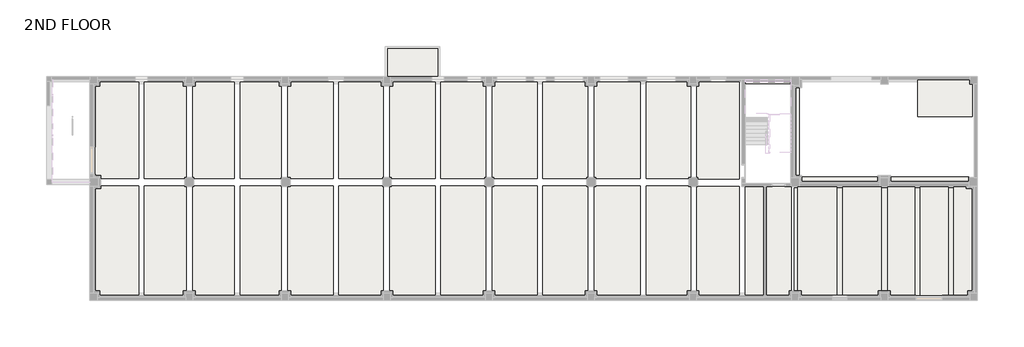
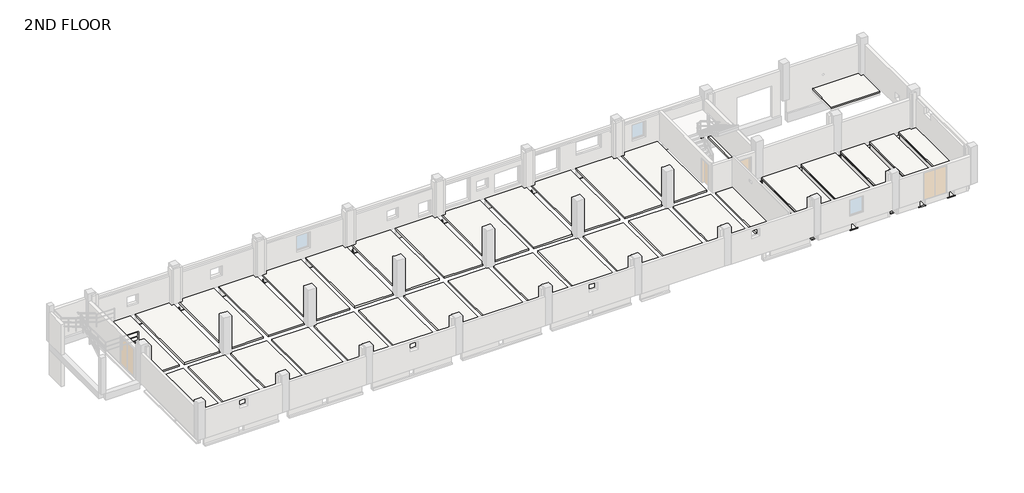
# One storey, part 4 of 7: 8 slabs, 2 coverings, 1 roof.
"""IFC4 building model written with IfcOpenShell, lengths in millimetres."""

from ifc_helpers import new_model, si_unit, frame, origin, place, context, project, spatial, polyline, outline, extrude, faceted_brep, element, save

model = new_model("IFC4")

# Units and contexts
model_context = context("Model", 3, world=origin())
ifc_project = project(units=[si_unit("LENGTHUNIT", "METRE", prefix="MILLI")], contexts=[model_context])

# Site, building, storey
site = spatial("IfcSite", under=ifc_project)
building = spatial("IfcBuilding", under=site)
storey = spatial("IfcBuildingStorey", under=building, Name="2ND FLOOR", Elevation=10600.0)

# Coverings
placement = place(None, origin())
element("IfcCovering", 1, ObjectType="H_CE_AR_B09_Souns Absorbing_100T_C7", at=placement, inside=storey, context=model_context, shape_type="SweptSolid", body=[
    extrude(outline(polyline([(58275.0, -8350.0), (58275.0, -16900.0), (55300.0, -16900.0), (55300.0, -16700.0), (55200.0, -16700.0), (55200.0, -8350.0), (58275.0, -8350.0)])), frame((0.0, 0.0, 10350.0), z_axis=(0.0, 0.0, 1.0), x_axis=(1.0, 0.0, 0.0)), (0.0, 0.0, 1.0), 100.0),
    extrude(outline(polyline([(58725.0, -8350.0), (61750.0, -8350.0), (61750.0, -16700.0), (61700.0, -16700.0), (61700.0, -16900.0), (58725.0, -16900.0), (58725.0, -8350.0)])), frame((0.0, 0.0, 10350.0), z_axis=(0.0, 0.0, 1.0), x_axis=(1.0, 0.0, 0.0)), (0.0, 0.0, 1.0), 100.0),
    extrude(outline(polyline([(64375.0, -8350.0), (64375.0, -16900.0), (62300.0, -16900.0), (62300.0, -16700.0), (62250.0, -16700.0), (62250.0, -8350.0), (64375.0, -8350.0)])), frame((0.0, 0.0, 10350.0), z_axis=(0.0, 0.0, 1.0), x_axis=(1.0, 0.0, 0.0)), (0.0, 0.0, 1.0), 100.0),
    extrude(outline(polyline([(67000.0, -8350.0), (67000.0, -16900.0), (64825.0, -16900.0), (64825.0, -8350.0), (67000.0, -8350.0)])), frame((0.0, 0.0, 10350.0), z_axis=(0.0, 0.0, 1.0), x_axis=(1.0, 0.0, 0.0)), (0.0, 0.0, 1.0), 100.0),
    extrude(outline(polyline([(68700.0, -16900.0), (67450.0, -16900.0), (67450.0, -8350.0), (68900.0, -8350.0), (68900.0, -16700.0), (68700.0, -16700.0), (68700.0, -16900.0)])), frame((0.0, 0.0, 10350.0), z_axis=(0.0, 0.0, 1.0), x_axis=(1.0, 0.0, 0.0)), (0.0, 0.0, 1.0), 100.0),
])
element("IfcCovering", 2, ObjectType="H_CE_AR_B09_Souns Absorbing_100T_C7", at=placement, inside=storey, context=model_context, shape_type="SweptSolid", body=[
    extrude(outline(polyline([(58175.0, -16886.0), (58175.0, -8469.0), (58825.0, -8469.0), (58825.0, -16886.0), (58175.0, -16886.0)])), frame((0.0, 0.0, 9700.0), z_axis=(0.0, 0.0, 1.0), x_axis=(1.0, 0.0, 0.0)), (0.0, 0.0, 1.0), 100.0),
    extrude(outline(polyline([(61650.0, -16536.0), (61650.0, -8469.0), (62350.0, -8469.0), (62350.0, -16536.0), (61650.0, -16536.0)])), frame((0.0, 0.0, 9700.0), z_axis=(0.0, 0.0, 1.0), x_axis=(1.0, 0.0, 0.0)), (0.0, 0.0, 1.0), 100.0),
    extrude(outline(polyline([(64275.0, -16886.0), (64275.0, -8469.0), (64925.0, -8469.0), (64925.0, -16886.0), (64275.0, -16886.0)])), frame((0.0, 0.0, 9700.0), z_axis=(0.0, 0.0, 1.0), x_axis=(1.0, 0.0, 0.0)), (0.0, 0.0, 1.0), 100.0),
    extrude(outline(polyline([(66900.0, -16886.0), (66900.0, -8469.0), (67550.0, -8469.0), (67550.0, -16886.0), (66900.0, -16886.0)])), frame((0.0, 0.0, 9700.0), z_axis=(0.0, 0.0, 1.0), x_axis=(1.0, 0.0, 0.0)), (0.0, 0.0, 1.0), 100.0),
    extrude(outline(polyline([(54937.0, -8469.0), (55300.0, -8469.0), (55300.0, -16536.0), (54937.0, -16536.0), (54937.0, -8469.0)])), frame((0.0, 0.0, 9700.0), z_axis=(0.0, 0.0, 1.0), x_axis=(1.0, 0.0, 0.0)), (0.0, 0.0, 1.0), 100.0),
])

# Roof
element("IfcRoof", 3, ObjectType="H_RF_AR_B06_RC Roof Finish_SkyPanel Roof_T160", at=placement, inside=storey, context=model_context, shape_type="SweptSolid", body=[
    extrude(outline(polyline([(23000.0, 2500.0), (27000.0, 2500.0), (27000.0, 300.0), (23000.0, 300.0), (23000.0, 2500.0)])), frame((0.0, 0.0, 9300.0), z_axis=(0.0, 0.0, 1.0), x_axis=(1.0, 0.0, 0.0)), (0.0, 0.0, 1.0), 170.0),
])

# Slabs
element("IfcSlab", 4, ObjectType="H_FL_AR_S17_RC Slab_T150_2S1", at=placement, inside=storey, context=model_context, shape_type="Brep", body=[
    faceted_brep([(3525.0, -100.0, 10450.0), (3525.0, -7700.0, 10450.0), (400.0, -7700.0, 10450.0), (399.4974747, -7700.0, 10450.0), (399.4974747, -7650.0, 10450.0), (100.0, -7650.0, 10450.0), (100.0, -300.0, 10450.0), (300.0, -300.0, 10450.0), (300.0, -100.0, 10450.0), (3525.0, -100.0, 10600.0), (300.0, -100.0, 10600.0), (300.0, -300.0, 10600.0), (100.0, -300.0, 10600.0), (100.0, -7650.0, 10600.0), (399.4974747, -7650.0, 10600.0), (399.4974747, -7700.0, 10600.0), (400.0, -7700.0, 10600.0), (3525.0, -7700.0, 10600.0)], [[[0, 1, 2, 3, 4, 5, 6, 7, 8]], [[9, 10, 11, 12, 13, 14, 15, 16, 17]], [[1, 0, 9, 17]], [[3, 2, 1, 17, 16, 15]], [[4, 3, 15, 14]], [[5, 4, 14, 13]], [[6, 5, 13, 12]], [[7, 6, 12, 11]], [[8, 7, 11, 10]], [[0, 8, 10, 9]]]),
    faceted_brep([(3975.0, -100.0, 10450.0), (7200.0, -100.0, 10450.0), (7200.0, -300.0, 10450.0), (7250.0, -300.0, 10450.0), (7250.0, -7650.0, 10450.0), (7150.0, -7650.0, 10450.0), (7150.0, -7700.0, 10450.0), (3975.0, -7700.0, 10450.0), (3975.0, -100.0, 10600.0), (3975.0, -7700.0, 10600.0), (7150.0, -7700.0, 10600.0), (7150.0, -7650.0, 10600.0), (7250.0, -7650.0, 10600.0), (7250.0, -300.0, 10600.0), (7200.0, -300.0, 10600.0), (7200.0, -100.0, 10600.0)], [[[0, 1, 2, 3, 4, 5, 6, 7]], [[8, 9, 10, 11, 12, 13, 14, 15]], [[1, 0, 8, 15]], [[2, 1, 15, 14]], [[3, 2, 14, 13]], [[4, 3, 13, 12]], [[5, 4, 12, 11]], [[6, 5, 11, 10]], [[7, 6, 10, 9]], [[0, 7, 9, 8]]]),
    faceted_brep([(3525.0, -16900.0, 10450.0), (300.0, -16900.0, 10450.0), (300.0, -16700.0, 10450.0), (100.0, -16700.0, 10450.0), (100.0, -8350.0, 10450.0), (399.4974747, -8350.0, 10450.0), (399.4974747, -8300.0, 10450.0), (400.0, -8300.0, 10450.0), (3525.0, -8300.0, 10450.0), (3525.0, -16900.0, 10600.0), (3525.0, -8300.0, 10600.0), (400.0, -8300.0, 10600.0), (399.4974747, -8300.0, 10600.0), (399.4974747, -8350.0, 10600.0), (100.0, -8350.0, 10600.0), (100.0, -16700.0, 10600.0), (300.0, -16700.0, 10600.0), (300.0, -16900.0, 10600.0)], [[[0, 1, 2, 3, 4, 5, 6, 7, 8]], [[9, 10, 11, 12, 13, 14, 15, 16, 17]], [[1, 0, 9, 17]], [[2, 1, 17, 16]], [[3, 2, 16, 15]], [[4, 3, 15, 14]], [[5, 4, 14, 13]], [[6, 5, 13, 12]], [[8, 7, 6, 12, 11, 10]], [[0, 8, 10, 9]]]),
    faceted_brep([(3975.0, -16900.0, 10450.0), (3975.0, -8300.0, 10450.0), (7150.0, -8300.0, 10450.0), (7150.0, -8350.0, 10450.0), (7250.0, -8350.0, 10450.0), (7250.0, -16700.0, 10450.0), (7200.0, -16700.0, 10450.0), (7200.0, -16900.0, 10450.0), (3975.0, -16900.0, 10600.0), (7200.0, -16900.0, 10600.0), (7200.0, -16700.0, 10600.0), (7250.0, -16700.0, 10600.0), (7250.0, -8350.0, 10600.0), (7150.0, -8350.0, 10600.0), (7150.0, -8300.0, 10600.0), (3975.0, -8300.0, 10600.0)], [[[0, 1, 2, 3, 4, 5, 6, 7]], [[8, 9, 10, 11, 12, 13, 14, 15]], [[1, 0, 8, 15]], [[2, 1, 15, 14]], [[3, 2, 14, 13]], [[4, 3, 13, 12]], [[5, 4, 12, 11]], [[6, 5, 11, 10]], [[7, 6, 10, 9]], [[0, 7, 9, 8]]]),
    faceted_brep([(11025.0, -100.0, 10450.0), (11025.0, -7700.0, 10450.0), (7850.0, -7700.0, 10450.0), (7850.0, -7650.0, 10450.0), (7750.0, -7650.0, 10450.0), (7750.0, -300.0, 10450.0), (7800.0, -300.0, 10450.0), (7800.0, -100.0, 10450.0), (11025.0, -100.0, 10600.0), (7800.0, -100.0, 10600.0), (7800.0, -300.0, 10600.0), (7750.0, -300.0, 10600.0), (7750.0, -7650.0, 10600.0), (7850.0, -7650.0, 10600.0), (7850.0, -7700.0, 10600.0), (11025.0, -7700.0, 10600.0)], [[[0, 1, 2, 3, 4, 5, 6, 7]], [[8, 9, 10, 11, 12, 13, 14, 15]], [[1, 0, 8, 15]], [[2, 1, 15, 14]], [[3, 2, 14, 13]], [[4, 3, 13, 12]], [[5, 4, 12, 11]], [[6, 5, 11, 10]], [[7, 6, 10, 9]], [[0, 7, 9, 8]]]),
    faceted_brep([(11025.0, -16900.0, 10450.0), (7800.0, -16900.0, 10450.0), (7800.0, -16700.0, 10450.0), (7750.0, -16700.0, 10450.0), (7750.0, -8350.0, 10450.0), (7850.0, -8350.0, 10450.0), (7850.0, -8300.0, 10450.0), (11025.0, -8300.0, 10450.0), (11025.0, -16900.0, 10600.0), (11025.0, -8300.0, 10600.0), (7850.0, -8300.0, 10600.0), (7850.0, -8350.0, 10600.0), (7750.0, -8350.0, 10600.0), (7750.0, -16700.0, 10600.0), (7800.0, -16700.0, 10600.0), (7800.0, -16900.0, 10600.0)], [[[0, 1, 2, 3, 4, 5, 6, 7]], [[8, 9, 10, 11, 12, 13, 14, 15]], [[1, 0, 8, 15]], [[2, 1, 15, 14]], [[3, 2, 14, 13]], [[4, 3, 13, 12]], [[5, 4, 12, 11]], [[6, 5, 11, 10]], [[7, 6, 10, 9]], [[0, 7, 9, 8]]]),
    faceted_brep([(14700.0, -100.0, 10450.0), (14700.0, -7700.0, 10450.0), (11475.0, -7700.0, 10450.0), (11475.0, -100.0, 10450.0), (14700.0, -100.0, 10600.0), (11475.0, -100.0, 10600.0), (11475.0, -7700.0, 10600.0), (14700.0, -7700.0, 10600.0), (14700.0, -7650.0, 10600.0), (14700.0, -300.0, 10600.0)], [[[0, 1, 2, 3]], [[4, 5, 6, 7, 8, 9]], [[1, 0, 4, 9, 8, 7]], [[2, 1, 7, 6]], [[3, 2, 6, 5]], [[0, 3, 5, 4]]]),
    faceted_brep([(11475.0, -8300.0, 10450.0), (14700.0, -8300.0, 10450.0), (14700.0, -16900.0, 10450.0), (11475.0, -16900.0, 10450.0), (11475.0, -8300.0, 10600.0), (11475.0, -16900.0, 10600.0), (14700.0, -16900.0, 10600.0), (14700.0, -16700.0, 10600.0), (14700.0, -8350.0, 10600.0), (14700.0, -8300.0, 10600.0)], [[[0, 1, 2, 3]], [[4, 5, 6, 7, 8, 9]], [[1, 0, 4, 9]], [[2, 1, 9, 8, 7, 6]], [[3, 2, 6, 5]], [[0, 3, 5, 4]]]),
    faceted_brep([(15300.0, -300.0, 10450.0), (15300.0, -100.0, 10450.0), (18775.0, -100.0, 10450.0), (18775.0, -7700.0, 10450.0), (15400.0000001, -7700.0, 10450.0), (15400.0000001, -7650.0, 10450.0), (15200.0, -7650.0, 10450.0), (15200.0, -300.0, 10450.0), (15300.0, -300.0, 10600.0), (15200.0, -300.0, 10600.0), (15200.0, -7650.0, 10600.0), (15400.0000001, -7650.0, 10600.0), (15400.0000001, -7700.0, 10600.0), (18775.0, -7700.0, 10600.0), (18775.0, -100.0, 10600.0), (15300.0, -100.0, 10600.0)], [[[0, 1, 2, 3, 4, 5, 6, 7]], [[8, 9, 10, 11, 12, 13, 14, 15]], [[1, 0, 8, 15]], [[2, 1, 15, 14]], [[3, 2, 14, 13]], [[4, 3, 13, 12]], [[5, 4, 12, 11]], [[6, 5, 11, 10]], [[7, 6, 10, 9]], [[0, 7, 9, 8]]]),
    faceted_brep([(15300.0, -16700.0, 10450.0), (15200.0, -16700.0, 10450.0), (15200.0, -8350.0, 10450.0), (15400.0000001, -8350.0, 10450.0), (15400.0000001, -8300.0, 10450.0), (18775.0, -8300.0, 10450.0), (18775.0, -16900.0, 10450.0), (15300.0, -16900.0, 10450.0), (15300.0, -16700.0, 10600.0), (15300.0, -16900.0, 10600.0), (18775.0, -16900.0, 10600.0), (18775.0, -8300.0, 10600.0), (15400.0000001, -8300.0, 10600.0), (15400.0000001, -8350.0, 10600.0), (15200.0, -8350.0, 10600.0), (15200.0, -16700.0, 10600.0)], [[[0, 1, 2, 3, 4, 5, 6, 7]], [[8, 9, 10, 11, 12, 13, 14, 15]], [[1, 0, 8, 15]], [[2, 1, 15, 14]], [[3, 2, 14, 13]], [[4, 3, 13, 12]], [[5, 4, 12, 11]], [[6, 5, 11, 10]], [[7, 6, 10, 9]], [[0, 7, 9, 8]]]),
    faceted_brep([(19225.0, -100.0, 10450.0), (22700.0, -100.0, 10450.0), (22700.0, -7650.0, 10450.0), (22650.0000003, -7650.0, 10450.0), (22650.0000003, -7700.0, 10450.0), (19225.0, -7700.0, 10450.0), (19225.0, -100.0, 10600.0), (19225.0, -7700.0, 10600.0), (22650.0000003, -7700.0, 10600.0), (22650.0000003, -7650.0, 10600.0), (22700.0, -7650.0, 10600.0), (22700.0, -300.0, 10600.0), (22700.0, -100.0, 10600.0)], [[[0, 1, 2, 3, 4, 5]], [[6, 7, 8, 9, 10, 11, 12]], [[1, 0, 6, 12]], [[2, 1, 12, 11, 10]], [[3, 2, 10, 9]], [[4, 3, 9, 8]], [[5, 4, 8, 7]], [[0, 5, 7, 6]]]),
    faceted_brep([(19225.0, -16900.0, 10450.0), (19225.0, -8300.0, 10450.0), (22650.0000003, -8300.0, 10450.0), (22650.0000003, -8350.0, 10450.0), (22700.0, -8350.0, 10450.0), (22700.0, -16900.0, 10450.0), (19225.0, -16900.0, 10600.0), (22700.0, -16900.0, 10600.0), (22700.0, -16700.0, 10600.0), (22700.0, -8350.0, 10600.0), (22650.0000003, -8350.0, 10600.0), (22650.0000003, -8300.0, 10600.0), (19225.0, -8300.0, 10600.0)], [[[0, 1, 2, 3, 4, 5]], [[6, 7, 8, 9, 10, 11, 12]], [[1, 0, 6, 12]], [[2, 1, 12, 11]], [[3, 2, 11, 10]], [[4, 3, 10, 9]], [[5, 4, 9, 8, 7]], [[0, 5, 7, 6]]]),
    faceted_brep([(23300.0, -100.0, 10450.0), (26775.0, -100.0, 10450.0), (26775.0, -7700.0, 10450.0), (23350.0000003, -7700.0, 10450.0), (23350.0000003, -7650.0, 10450.0), (23200.0, -7650.0, 10450.0), (23200.0, -300.0, 10450.0), (23300.0, -300.0, 10450.0), (23300.0, -100.0, 10600.0), (23300.0, -300.0, 10600.0), (23200.0, -300.0, 10600.0), (23200.0, -7650.0, 10600.0), (23350.0000003, -7650.0, 10600.0), (23350.0000003, -7700.0, 10600.0), (26775.0, -7700.0, 10600.0), (26775.0, -100.0, 10600.0)], [[[0, 1, 2, 3, 4, 5, 6, 7]], [[8, 9, 10, 11, 12, 13, 14, 15]], [[1, 0, 8, 15]], [[2, 1, 15, 14]], [[3, 2, 14, 13]], [[4, 3, 13, 12]], [[5, 4, 12, 11]], [[6, 5, 11, 10]], [[7, 6, 10, 9]], [[0, 7, 9, 8]]]),
    faceted_brep([(23300.0, -16900.0, 10450.0), (23300.0, -16700.0, 10450.0), (23200.0, -16700.0, 10450.0), (23200.0, -8350.0, 10450.0), (23350.0000003, -8350.0, 10450.0), (23350.0000003, -8300.0, 10450.0), (26775.0, -8300.0, 10450.0), (26775.0, -16900.0, 10450.0), (23300.0, -16900.0, 10600.0), (26775.0, -16900.0, 10600.0), (26775.0, -8300.0, 10600.0), (23350.0000003, -8300.0, 10600.0), (23350.0000003, -8350.0, 10600.0), (23200.0, -8350.0, 10600.0), (23200.0, -16700.0, 10600.0), (23300.0, -16700.0, 10600.0)], [[[0, 1, 2, 3, 4, 5, 6, 7]], [[8, 9, 10, 11, 12, 13, 14, 15]], [[1, 0, 8, 15]], [[2, 1, 15, 14]], [[3, 2, 14, 13]], [[4, 3, 13, 12]], [[5, 4, 12, 11]], [[6, 5, 11, 10]], [[7, 6, 10, 9]], [[0, 7, 9, 8]]]),
    faceted_brep([(30700.0, -100.0, 10450.0), (30700.0, -300.0, 10450.0), (30750.0000002, -300.0, 10450.0), (30750.0000002, -7650.0, 10450.0), (30649.9999997, -7650.0, 10450.0), (30649.9999997, -7700.0, 10450.0), (27225.0, -7700.0, 10450.0), (27225.0, -100.0, 10450.0), (30700.0, -100.0, 10600.0), (27225.0, -100.0, 10600.0), (27225.0, -7700.0, 10600.0), (30649.9999997, -7700.0, 10600.0), (30649.9999997, -7650.0, 10600.0), (30750.0000002, -7650.0, 10600.0), (30750.0000002, -300.0, 10600.0), (30700.0, -300.0, 10600.0)], [[[0, 1, 2, 3, 4, 5, 6, 7]], [[8, 9, 10, 11, 12, 13, 14, 15]], [[1, 0, 8, 15]], [[2, 1, 15, 14]], [[3, 2, 14, 13]], [[4, 3, 13, 12]], [[5, 4, 12, 11]], [[6, 5, 11, 10]], [[7, 6, 10, 9]], [[0, 7, 9, 8]]]),
    faceted_brep([(30700.0, -16900.0, 10450.0), (27225.0, -16900.0, 10450.0), (27225.0, -8300.0, 10450.0), (30649.9999997, -8300.0, 10450.0), (30649.9999997, -8350.0, 10450.0), (30750.0000002, -8350.0, 10450.0), (30750.0000002, -16700.0, 10450.0), (30700.0, -16700.0, 10450.0), (30700.0, -16900.0, 10600.0), (30700.0, -16700.0, 10600.0), (30750.0000002, -16700.0, 10600.0), (30750.0000002, -8350.0, 10600.0), (30649.9999997, -8350.0, 10600.0), (30649.9999997, -8300.0, 10600.0), (27225.0, -8300.0, 10600.0), (27225.0, -16900.0, 10600.0)], [[[0, 1, 2, 3, 4, 5, 6, 7]], [[8, 9, 10, 11, 12, 13, 14, 15]], [[1, 0, 8, 15]], [[2, 1, 15, 14]], [[3, 2, 14, 13]], [[4, 3, 13, 12]], [[5, 4, 12, 11]], [[6, 5, 11, 10]], [[7, 6, 10, 9]], [[0, 7, 9, 8]]]),
    faceted_brep([(31300.0, -100.0, 10450.0), (34775.0, -100.0, 10450.0), (34775.0, -7700.0, 10450.0), (31350.0000003, -7700.0, 10450.0), (31350.0000003, -7650.0, 10450.0), (31249.9999998, -7650.0, 10450.0), (31249.9999998, -300.0, 10450.0), (31300.0, -300.0, 10450.0), (31300.0, -100.0, 10600.0), (31300.0, -300.0, 10600.0), (31249.9999998, -300.0, 10600.0), (31249.9999998, -7650.0, 10600.0), (31350.0000003, -7650.0, 10600.0), (31350.0000003, -7700.0, 10600.0), (34775.0, -7700.0, 10600.0), (34775.0, -100.0, 10600.0)], [[[0, 1, 2, 3, 4, 5, 6, 7]], [[8, 9, 10, 11, 12, 13, 14, 15]], [[1, 0, 8, 15]], [[2, 1, 15, 14]], [[3, 2, 14, 13]], [[4, 3, 13, 12]], [[5, 4, 12, 11]], [[6, 5, 11, 10]], [[7, 6, 10, 9]], [[0, 7, 9, 8]]]),
    faceted_brep([(31300.0, -16900.0, 10450.0), (31300.0, -16700.0, 10450.0), (31249.9999998, -16700.0, 10450.0), (31249.9999998, -8350.0, 10450.0), (31350.0000003, -8350.0, 10450.0), (31350.0000003, -8300.0, 10450.0), (34775.0, -8300.0, 10450.0), (34775.0, -16900.0, 10450.0), (31300.0, -16900.0, 10600.0), (34775.0, -16900.0, 10600.0), (34775.0, -8300.0, 10600.0), (31350.0000003, -8300.0, 10600.0), (31350.0000003, -8350.0, 10600.0), (31249.9999998, -8350.0, 10600.0), (31249.9999998, -16700.0, 10600.0), (31300.0, -16700.0, 10600.0)], [[[0, 1, 2, 3, 4, 5, 6, 7]], [[8, 9, 10, 11, 12, 13, 14, 15]], [[1, 0, 8, 15]], [[2, 1, 15, 14]], [[3, 2, 14, 13]], [[4, 3, 13, 12]], [[5, 4, 12, 11]], [[6, 5, 11, 10]], [[7, 6, 10, 9]], [[0, 7, 9, 8]]]),
    faceted_brep([(38700.0, -100.0, 10450.0), (38700.0, -300.0, 10450.0), (38750.0000002, -300.0, 10450.0), (38750.0000002, -7650.0, 10450.0), (38649.9999997, -7650.0, 10450.0), (38649.9999997, -7700.0, 10450.0), (35225.0, -7700.0, 10450.0), (35225.0, -100.0, 10450.0), (38700.0, -100.0, 10600.0), (35225.0, -100.0, 10600.0), (35225.0, -7700.0, 10600.0), (38649.9999997, -7700.0, 10600.0), (38649.9999997, -7650.0, 10600.0), (38750.0000002, -7650.0, 10600.0), (38750.0000002, -300.0, 10600.0), (38700.0, -300.0, 10600.0)], [[[0, 1, 2, 3, 4, 5, 6, 7]], [[8, 9, 10, 11, 12, 13, 14, 15]], [[1, 0, 8, 15]], [[2, 1, 15, 14]], [[3, 2, 14, 13]], [[4, 3, 13, 12]], [[5, 4, 12, 11]], [[6, 5, 11, 10]], [[7, 6, 10, 9]], [[0, 7, 9, 8]]]),
    faceted_brep([(38700.0, -16900.0, 10450.0), (35225.0, -16900.0, 10450.0), (35225.0, -8300.0, 10450.0), (38649.9999997, -8300.0, 10450.0), (38649.9999997, -8350.0, 10450.0), (38750.0000002, -8350.0, 10450.0), (38750.0000002, -16700.0, 10450.0), (38700.0, -16700.0, 10450.0), (38700.0, -16900.0, 10600.0), (38700.0, -16700.0, 10600.0), (38750.0000002, -16700.0, 10600.0), (38750.0000002, -8350.0, 10600.0), (38649.9999997, -8350.0, 10600.0), (38649.9999997, -8300.0, 10600.0), (35225.0, -8300.0, 10600.0), (35225.0, -16900.0, 10600.0)], [[[0, 1, 2, 3, 4, 5, 6, 7]], [[8, 9, 10, 11, 12, 13, 14, 15]], [[1, 0, 8, 15]], [[2, 1, 15, 14]], [[3, 2, 14, 13]], [[4, 3, 13, 12]], [[5, 4, 12, 11]], [[6, 5, 11, 10]], [[7, 6, 10, 9]], [[0, 7, 9, 8]]]),
    faceted_brep([(39300.0, -100.0, 10450.0), (42875.0, -100.0, 10450.0), (42875.0, -7700.0, 10450.0), (39350.0000003, -7700.0, 10450.0), (39350.0000003, -7650.0, 10450.0), (39249.9999998, -7650.0, 10450.0), (39249.9999998, -300.0, 10450.0), (39300.0, -300.0, 10450.0), (39300.0, -100.0, 10600.0), (39300.0, -300.0, 10600.0), (39249.9999998, -300.0, 10600.0), (39249.9999998, -7650.0, 10600.0), (39350.0000003, -7650.0, 10600.0), (39350.0000003, -7700.0, 10600.0), (42875.0, -7700.0, 10600.0), (42875.0, -100.0, 10600.0)], [[[0, 1, 2, 3, 4, 5, 6, 7]], [[8, 9, 10, 11, 12, 13, 14, 15]], [[1, 0, 8, 15]], [[2, 1, 15, 14]], [[3, 2, 14, 13]], [[4, 3, 13, 12]], [[5, 4, 12, 11]], [[6, 5, 11, 10]], [[7, 6, 10, 9]], [[0, 7, 9, 8]]]),
    faceted_brep([(39300.0, -16900.0, 10450.0), (39300.0, -16700.0, 10450.0), (39249.9999998, -16700.0, 10450.0), (39249.9999998, -8350.0, 10450.0), (39350.0000003, -8350.0, 10450.0), (39350.0000003, -8300.0, 10450.0), (42875.0, -8300.0, 10450.0), (42875.0, -16900.0, 10450.0), (39300.0, -16900.0, 10600.0), (42875.0, -16900.0, 10600.0), (42875.0, -8300.0, 10600.0), (39350.0000003, -8300.0, 10600.0), (39350.0000003, -8350.0, 10600.0), (39249.9999998, -8350.0, 10600.0), (39249.9999998, -16700.0, 10600.0), (39300.0, -16700.0, 10600.0)], [[[0, 1, 2, 3, 4, 5, 6, 7]], [[8, 9, 10, 11, 12, 13, 14, 15]], [[1, 0, 8, 15]], [[2, 1, 15, 14]], [[3, 2, 14, 13]], [[4, 3, 13, 12]], [[5, 4, 12, 11]], [[6, 5, 11, 10]], [[7, 6, 10, 9]], [[0, 7, 9, 8]]]),
    faceted_brep([(46700.0, -100.0, 10450.0), (46700.0, -300.0, 10450.0), (46800.0, -300.0, 10450.0), (46800.0, -7650.0, 10450.0), (46649.9999999, -7650.0, 10450.0), (46649.9999999, -7700.0, 10450.0), (43325.0, -7700.0, 10450.0), (43325.0, -100.0, 10450.0), (46700.0, -100.0, 10600.0), (43325.0, -100.0, 10600.0), (43325.0, -7700.0, 10600.0), (46649.9999999, -7700.0, 10600.0), (46649.9999999, -7650.0, 10600.0), (46800.0, -7650.0, 10600.0), (46800.0, -300.0, 10600.0), (46700.0, -300.0, 10600.0)], [[[0, 1, 2, 3, 4, 5, 6, 7]], [[8, 9, 10, 11, 12, 13, 14, 15]], [[1, 0, 8, 15]], [[2, 1, 15, 14]], [[3, 2, 14, 13]], [[4, 3, 13, 12]], [[5, 4, 12, 11]], [[6, 5, 11, 10]], [[7, 6, 10, 9]], [[0, 7, 9, 8]]]),
    faceted_brep([(46700.0, -16900.0, 10450.0), (43325.0, -16900.0, 10450.0), (43325.0, -8300.0, 10450.0), (46649.9999999, -8300.0, 10450.0), (46649.9999999, -8350.0, 10450.0), (46800.0, -8350.0, 10450.0), (46800.0, -16700.0, 10450.0), (46700.0, -16700.0, 10450.0), (46700.0, -16900.0, 10600.0), (46700.0, -16700.0, 10600.0), (46800.0, -16700.0, 10600.0), (46800.0, -8350.0, 10600.0), (46649.9999999, -8350.0, 10600.0), (46649.9999999, -8300.0, 10600.0), (43325.0, -8300.0, 10600.0), (43325.0, -16900.0, 10600.0)], [[[0, 1, 2, 3, 4, 5, 6, 7]], [[8, 9, 10, 11, 12, 13, 14, 15]], [[1, 0, 8, 15]], [[2, 1, 15, 14]], [[3, 2, 14, 13]], [[4, 3, 13, 12]], [[5, 4, 12, 11]], [[6, 5, 11, 10]], [[7, 6, 10, 9]], [[0, 7, 9, 8]]]),
    faceted_brep([(50625.0, -8350.0, 10450.0), (50625.0, -16900.0, 10450.0), (47300.0, -16900.0, 10450.0), (47300.0, -8350.0, 10450.0), (50625.0, -8350.0, 10600.0), (47349.9999999, -8350.0, 10600.0), (47300.0, -8350.0, 10600.0), (47300.0, -16700.0, 10600.0), (47300.0, -16900.0, 10600.0), (50625.0, -16900.0, 10600.0)], [[[0, 1, 2, 3]], [[4, 5, 6, 7, 8, 9]], [[1, 0, 4, 9]], [[2, 1, 9, 8]], [[3, 2, 8, 7, 6]], [[0, 3, 6, 5, 4]]]),
    faceted_brep([(50625.0, -100.0, 10450.0), (50625.0, -7750.0, 10450.0), (47349.9999999, -7750.0, 10450.0), (47349.9999999, -7650.0, 10450.0), (47300.0, -7650.0, 10450.0), (47300.0, -100.0, 10450.0), (50625.0, -100.0, 10600.0), (47300.0, -100.0, 10600.0), (47300.0, -300.0, 10600.0), (47300.0, -7650.0, 10600.0), (47349.9999999, -7650.0, 10600.0), (47349.9999999, -7750.0, 10600.0), (50625.0, -7750.0, 10600.0)], [[[0, 1, 2, 3, 4, 5]], [[6, 7, 8, 9, 10, 11, 12]], [[1, 0, 6, 12]], [[2, 1, 12, 11]], [[3, 2, 11, 10]], [[4, 3, 10, 9]], [[5, 4, 9, 8, 7]], [[0, 5, 7, 6]]]),
    faceted_brep([(54700.0, -8350.0, 10450.0), (54700.0, -16900.0, 10450.0), (51075.0, -16900.0, 10450.0), (51075.0, -8350.0, 10450.0), (54700.0, -8350.0, 10600.0), (54650.0, -8350.0, 10600.0), (51075.0, -8350.0, 10600.0), (51075.0, -16900.0, 10600.0), (54700.0, -16900.0, 10600.0), (54700.0, -16700.0, 10600.0)], [[[0, 1, 2, 3]], [[4, 5, 6, 7, 8, 9]], [[1, 0, 4, 9, 8]], [[2, 1, 8, 7]], [[3, 2, 7, 6]], [[0, 3, 6, 5, 4]]]),
    faceted_brep([(58275.0, -8350.0, 10450.0), (58275.0, -16900.0, 10450.0), (55300.0, -16900.0, 10450.0), (55300.0, -16700.0, 10450.0), (55200.0, -16700.0, 10450.0), (55200.0, -8350.0, 10450.0), (58275.0, -8350.0, 10600.0), (55350.0, -8350.0, 10600.0), (55200.0, -8350.0, 10600.0), (55200.0, -16700.0, 10600.0), (55300.0, -16700.0, 10600.0), (55300.0, -16900.0, 10600.0), (58275.0, -16900.0, 10600.0)], [[[0, 1, 2, 3, 4, 5]], [[6, 7, 8, 9, 10, 11, 12]], [[1, 0, 6, 12]], [[2, 1, 12, 11]], [[3, 2, 11, 10]], [[4, 3, 10, 9]], [[5, 4, 9, 8]], [[0, 5, 8, 7, 6]]]),
    faceted_brep([(58725.0, -8350.0, 10450.0), (61750.0, -8350.0, 10450.0), (61750.0, -16700.0, 10450.0), (61700.0, -16700.0, 10450.0), (61700.0, -16900.0, 10450.0), (58725.0, -16900.0, 10450.0), (58725.0, -8350.0, 10600.0), (58725.0, -16900.0, 10600.0), (61700.0, -16900.0, 10600.0), (61700.0, -16700.0, 10600.0), (61750.0, -16700.0, 10600.0), (61750.0, -8350.0, 10600.0), (61650.0, -8350.0, 10600.0)], [[[0, 1, 2, 3, 4, 5]], [[6, 7, 8, 9, 10, 11, 12]], [[1, 0, 6, 12, 11]], [[2, 1, 11, 10]], [[3, 2, 10, 9]], [[4, 3, 9, 8]], [[5, 4, 8, 7]], [[0, 5, 7, 6]]]),
    faceted_brep([(64375.0, -8350.0, 10450.0), (64375.0, -16900.0, 10450.0), (62300.0, -16900.0, 10450.0), (62300.0, -16700.0, 10450.0), (62250.0, -16700.0, 10450.0), (62250.0, -8350.0, 10450.0), (64375.0, -8350.0, 10600.0), (62350.0, -8350.0, 10600.0), (62250.0, -8350.0, 10600.0), (62250.0, -16700.0, 10600.0), (62300.0, -16700.0, 10600.0), (62300.0, -16900.0, 10600.0), (64375.0, -16900.0, 10600.0)], [[[0, 1, 2, 3, 4, 5]], [[6, 7, 8, 9, 10, 11, 12]], [[1, 0, 6, 12]], [[2, 1, 12, 11]], [[3, 2, 11, 10]], [[4, 3, 10, 9]], [[5, 4, 9, 8]], [[0, 5, 8, 7, 6]]]),
    faceted_brep([(67000.0, -8350.0, 10450.0), (67000.0, -16900.0, 10450.0), (64825.0, -16900.0, 10450.0), (64825.0, -8350.0, 10450.0), (67000.0, -8350.0, 10600.0), (64825.0, -8350.0, 10600.0), (64825.0, -16900.0, 10600.0), (67000.0, -16900.0, 10600.0)], [[[0, 1, 2, 3]], [[4, 5, 6, 7]], [[1, 0, 4, 7]], [[2, 1, 7, 6]], [[3, 2, 6, 5]], [[0, 3, 5, 4]]]),
    faceted_brep([(68700.0, -16900.0, 10450.0), (67450.0, -16900.0, 10450.0), (67450.0, -8350.0, 10450.0), (68900.0, -8350.0, 10450.0), (68900.0, -16700.0, 10450.0), (68700.0, -16700.0, 10450.0), (68700.0, -16900.0, 10600.0), (68700.0, -16700.0, 10600.0), (68900.0, -16700.0, 10600.0), (68900.0, -8350.0, 10600.0), (68600.0, -8350.0, 10600.0), (67450.0, -8350.0, 10600.0), (67450.0, -16900.0, 10600.0)], [[[0, 1, 2, 3, 4, 5]], [[6, 7, 8, 9, 10, 11, 12]], [[1, 0, 6, 12]], [[2, 1, 12, 11]], [[3, 2, 11, 10, 9]], [[4, 3, 9, 8]], [[5, 4, 8, 7]], [[0, 5, 7, 6]]]),
])
element("IfcSlab", 5, ObjectType="H_FL_AR_S17_RC Slab_T150_2S2", at=placement, inside=storey, context=model_context, shape_type="SweptSolid", body=[
    extrude(outline(polyline([(68900.0, -2850.0), (64600.0, -2850.0), (64600.0, 50.0), (68700.0, 50.0), (68700.0, -300.0), (68900.0, -300.0), (68900.0, -2850.0)])), frame((0.0, 0.0, 10450.0), z_axis=(0.0, 0.0, 1.0), x_axis=(1.0, 0.0, 0.0)), (0.0, 0.0, 1.0), 150.0),
])
element("IfcSlab", 6, ObjectType="H_FL_AR_S17_RC Slab_T150_2CS1", at=placement, inside=storey, context=model_context, shape_type="SweptSolid", body=[
    extrude(outline(polyline([(26850.0, 2350.0), (26850.0, 300.0), (23150.0, 300.0), (23150.0, 2350.0), (26850.0, 2350.0)])), frame((0.0, 0.0, 9150.0), z_axis=(0.0, 0.0, 1.0), x_axis=(1.0, 0.0, 0.0)), (0.0, 0.0, 1.0), 150.0),
])
element("IfcSlab", 7, ObjectType="H_FL_AR_B07l_2L Gypsum_Insulationl_T154", at=placement, inside=storey, context=model_context, shape_type="Brep", body=[
    faceted_brep([(54910.0, -7486.0, 10600.0), (54910.0, -564.0, 10600.0), (55160.0, -564.0, 10600.0), (55160.0, -7486.0, 10600.0), (55314.0, -564.0, 10754.0), (55064.0, -564.0, 10754.0), (54910.0, -564.0, 10754.0), (54910.0, -7486.0, 10754.0), (55064.0, -7486.0, 10754.0), (55314.0, -7486.0, 10754.0), (55314.0, -564.0, 10735.0), (55160.0, -564.0, 10735.0), (55314.0, -7486.0, 10735.0), (54910.0, -7486.0, 10735.0), (55160.0, -7486.0, 10735.0)], [[[0, 1, 2, 3]], [[4, 5, 6, 7, 8, 9]], [[6, 5, 4, 10, 11, 2, 1]], [[4, 9, 12, 10]], [[9, 8, 7, 13, 0, 3, 14, 12]], [[1, 0, 13, 7, 6]], [[11, 14, 3, 2]], [[14, 11, 10, 12]]]),
    faceted_brep([(61486.0, -8090.0, 10600.0), (55514.0, -8090.0, 10600.0), (55514.0, -7740.0, 10600.0), (61486.0, -7740.0, 10600.0), (61486.0, -8090.0, 10754.0), (61486.0, -7936.0, 10754.0), (61486.0, -7586.0, 10754.0), (55514.0, -7586.0, 10754.0), (55514.0, -7936.0, 10754.0), (55514.0, -8090.0, 10754.0), (61486.0, -8090.0, 10735.0), (61486.0, -7740.0, 10735.0), (61486.0, -7586.0, 10735.0), (55514.0, -8090.0, 10735.0), (55514.0, -7586.0, 10735.0), (55514.0, -7740.0, 10735.0)], [[[0, 1, 2, 3]], [[4, 5, 6, 7, 8, 9]], [[6, 5, 4, 10, 0, 3, 11, 12]], [[1, 0, 10, 4, 9, 13]], [[9, 8, 7, 14, 15, 2, 1, 13]], [[7, 6, 12, 14]], [[15, 11, 3, 2]], [[11, 15, 14, 12]]]),
    faceted_brep([(68600.0, -8090.0, 10600.0), (62514.0, -8090.0, 10600.0), (62514.0, -7740.0, 10600.0), (68600.0, -7740.0, 10600.0), (68600.0, -8090.0, 10754.0), (68600.0, -7936.0, 10754.0), (68600.0, -7586.0, 10754.0), (62514.0, -7586.0, 10754.0), (62514.0, -7936.0, 10754.0), (62514.0, -8090.0, 10754.0), (68600.0, -7740.0, 10735.0), (68600.0, -7586.0, 10735.0), (62514.0, -7586.0, 10735.0), (62514.0, -7740.0, 10735.0)], [[[0, 1, 2, 3]], [[4, 5, 6, 7, 8, 9]], [[6, 5, 4, 0, 3, 10, 11]], [[1, 0, 4, 9]], [[9, 8, 7, 12, 13, 2, 1]], [[7, 6, 11, 12]], [[13, 10, 3, 2]], [[10, 13, 12, 11]]]),
])
element("IfcSlab", 8, ObjectType="H_WA_AR_B02_Int Wall_2L Gypsum_Insulationl_T154(Mirror)", at=placement, inside=storey, context=model_context, shape_type="Brep", body=[
    faceted_brep([(54910.0, -564.0, 9646.0), (55064.0, -564.0, 9646.0), (55314.0, -564.0, 9646.0), (55314.0, -7486.0, 9646.0), (55064.0, -7486.0, 9646.0), (54910.0, -7486.0, 9646.0), (54910.0, -564.0, 9800.0), (54910.0, -7486.0, 9800.0), (55160.0, -7486.0, 9800.0), (55160.0, -564.0, 9800.0), (55160.0, -564.0, 9665.0), (55314.0, -564.0, 9665.0), (55314.0, -7486.0, 9665.0), (55160.0, -7486.0, 9665.0), (54910.0, -7486.0, 9665.0)], [[[0, 1, 2, 3, 4, 5]], [[6, 7, 8, 9]], [[2, 1, 0, 6, 9, 10, 11]], [[3, 2, 11, 12]], [[5, 4, 3, 12, 13, 8, 7, 14]], [[0, 5, 14, 7, 6]], [[13, 10, 9, 8]], [[10, 13, 12, 11]]]),
    faceted_brep([(61486.0, -7586.0, 9646.0), (61486.0, -7936.0, 9646.0), (61486.0, -8090.0, 9646.0), (55514.0, -8090.0, 9646.0), (55514.0, -7936.0, 9646.0), (55514.0, -7586.0, 9646.0), (55514.0, -8090.0, 9800.0), (61486.0, -8090.0, 9800.0), (61486.0, -7740.0, 9800.0), (55514.0, -7740.0, 9800.0), (61486.0, -7586.0, 9665.0), (61486.0, -7740.0, 9665.0), (61486.0, -8090.0, 9665.0), (55514.0, -8090.0, 9665.0), (55514.0, -7740.0, 9665.0), (55514.0, -7586.0, 9665.0)], [[[0, 1, 2, 3, 4, 5]], [[6, 7, 8, 9]], [[2, 1, 0, 10, 11, 8, 7, 12]], [[3, 2, 12, 7, 6, 13]], [[5, 4, 3, 13, 6, 9, 14, 15]], [[0, 5, 15, 10]], [[11, 14, 9, 8]], [[14, 11, 10, 15]]]),
    faceted_brep([(68600.0, -7586.0, 9646.0), (68600.0, -7936.0, 9646.0), (68600.0, -8090.0, 9646.0), (62514.0, -8090.0, 9646.0), (62514.0, -7936.0, 9646.0), (62514.0, -7586.0, 9646.0), (62514.0, -8090.0, 9800.0), (68600.0, -8090.0, 9800.0), (68600.0, -7740.0, 9800.0), (62514.0, -7740.0, 9800.0), (68600.0, -7586.0, 9665.0), (68600.0, -7740.0, 9665.0), (62514.0, -7740.0, 9665.0), (62514.0, -7586.0, 9665.0)], [[[0, 1, 2, 3, 4, 5]], [[6, 7, 8, 9]], [[2, 1, 0, 10, 11, 8, 7]], [[3, 2, 7, 6]], [[5, 4, 3, 6, 9, 12, 13]], [[0, 5, 13, 10]], [[11, 12, 9, 8]], [[12, 11, 10, 13]]]),
])
element("IfcSlab", 9, ObjectType="H_WA_AR_B02_Int Wall_2L Gypsum_Insulationl_T154(Mirror)", at=placement, inside=storey, context=model_context, shape_type="Brep", body=[
    faceted_brep([(54650.0, -264.0, 9636.0), (51074.7487373, -264.0, 9636.0), (51074.7487373, 40.0, 9636.0), (51075.0, 40.0, 9636.0), (54650.0, 40.0, 9636.0), (54650.0, -114.0, 9636.0), (54650.0, 40.0, 9790.0), (51074.7487373, 40.0, 9790.0), (51074.7487373, -110.0, 9790.0), (54650.0, -110.0, 9790.0), (54650.0, -264.0, 9655.0), (51074.7487373, -264.0, 9655.0), (51074.7487373, -110.0, 9655.0), (54650.0, -110.0, 9655.0)], [[[0, 1, 2, 3, 4, 5]], [[6, 7, 8, 9]], [[1, 0, 10, 11]], [[2, 1, 11, 12, 8, 7]], [[4, 3, 2, 7, 6]], [[0, 5, 4, 6, 9, 13, 10]], [[12, 13, 9, 8]], [[13, 12, 11, 10]]]),
])
element("IfcSlab", 10, ObjectType="H_FL_AR_B07l_2L Gypsum_Insulationl_T154", at=placement, inside=storey, context=model_context, shape_type="Brep", body=[
    faceted_brep([(51074.7487373, 40.0, 10610.0), (54650.0, 40.0, 10610.0), (54650.0, -110.0, 10610.0), (51074.7487373, -110.0, 10610.0), (51074.7487373, -264.0, 10764.0), (54650.0, -264.0, 10764.0), (54650.0, -114.0, 10764.0), (54650.0, 40.0, 10764.0), (51074.7487373, 40.0, 10764.0), (51074.7487373, -114.0, 10764.0), (51074.7487373, -264.0, 10735.0), (54650.0, -264.0, 10735.0), (51074.7487373, -110.0, 10735.0), (54650.0, -110.0, 10735.0)], [[[0, 1, 2, 3]], [[4, 5, 6, 7, 8, 9]], [[5, 4, 10, 11]], [[4, 9, 8, 0, 3, 12, 10]], [[1, 0, 8, 7]], [[7, 6, 5, 11, 13, 2, 1]], [[13, 12, 3, 2]], [[12, 13, 11, 10]]]),
])
element("IfcSlab", 11, ObjectType="H_WA_AR_B02_Int Wall_2L Gypsum_Insulationl_T154(Mirror)", at=placement, inside=storey, context=model_context, shape_type="Brep", body=[
    faceted_brep([(2201.0, -264.0, 9636.0), (464.0, -264.0, 9636.0), (464.0, -114.0, 9636.0), (2201.0, -114.0, 9636.0), (464.0, -264.0, 9655.0), (464.0, -114.0, 9655.0), (2201.0, -264.0, 9655.0), (2201.0, -114.0, 9655.0)], [[[0, 1, 2, 3]], [[1, 4, 5, 2]], [[1, 0, 6, 4]], [[4, 6, 7, 5]], [[3, 2, 5, 7]], [[6, 0, 3, 7]]]),
    faceted_brep([(14536.0, -264.0, 9636.0), (7964.0, -264.0, 9636.0), (7964.0, -114.0, 9636.0), (14536.0, -114.0, 9636.0), (14536.0, -264.0, 9655.0), (14536.0, -114.0, 9655.0), (7964.0, -264.0, 9655.0), (7964.0, -114.0, 9655.0)], [[[0, 1, 2, 3]], [[4, 0, 3, 5]], [[1, 6, 7, 2]], [[1, 0, 4, 6]], [[6, 4, 5, 7]], [[3, 2, 7, 5]]]),
    faceted_brep([(7036.0, -114.0, 9636.0), (7036.0, -264.0, 9636.0), (2329.0, -264.0, 9636.0), (2329.0, -114.0, 9636.0), (7036.0, -114.0, 9655.0), (7036.0, -264.0, 9655.0), (2329.0, -114.0, 9655.0), (2329.0, -264.0, 9655.0)], [[[0, 1, 2, 3]], [[1, 0, 4, 5]], [[4, 0, 3, 6]], [[2, 1, 5, 7]], [[3, 2, 7, 6]], [[5, 4, 6, 7]]]),
    faceted_brep([(43325.0, -264.0, 9636.0), (43325.0, 40.0, 9636.0), (46536.0, 40.0, 9636.0), (46536.0, -264.0, 9636.0), (46536.0, 40.0, 9790.0), (43325.0, 40.0, 9790.0), (43325.0, -110.0, 9790.0), (46536.0, -110.0, 9790.0), (43325.0, -264.0, 9655.0), (43325.0, -110.0, 9655.0), (46536.0, -110.0, 9655.0), (46536.0, -264.0, 9655.0)], [[[0, 1, 2, 3]], [[4, 5, 6, 7]], [[1, 0, 8, 9, 6, 5]], [[2, 1, 5, 4]], [[3, 2, 4, 7, 10, 11]], [[0, 3, 11, 8]], [[9, 10, 7, 6]], [[10, 9, 8, 11]]]),
    faceted_brep([(15464.0, 40.0, 9636.0), (22536.0, 40.0, 9636.0), (22536.0, -114.0, 9636.0), (22536.0, -264.0, 9636.0), (15464.0, -264.0, 9636.0), (15464.0, -114.0, 9636.0), (22536.0, 40.0, 9790.0), (15464.0, 40.0, 9790.0), (15464.0, -110.0, 9790.0), (22536.0, -110.0, 9790.0), (15464.0, -264.0, 9655.0), (15464.0, -110.0, 9655.0), (22536.0, -264.0, 9655.0), (22536.0, -110.0, 9655.0)], [[[0, 1, 2, 3, 4, 5]], [[6, 7, 8, 9]], [[1, 0, 7, 6]], [[0, 5, 4, 10, 11, 8, 7]], [[4, 3, 12, 10]], [[3, 2, 1, 6, 9, 13, 12]], [[11, 13, 9, 8]], [[13, 11, 10, 12]]]),
    faceted_brep([(23464.0, -264.0, 9636.0), (23464.0, -114.0, 9636.0), (23464.0, 40.0, 9636.0), (26907.0, 40.0, 9636.0), (30536.0, 40.0, 9636.0), (30536.0, -264.0, 9636.0), (30536.0, 40.0, 9790.0), (23464.0, 40.0, 9790.0), (23464.0, -110.0, 9790.0), (30536.0, -110.0, 9790.0), (23464.0, -264.0, 9655.0), (23464.0, -110.0, 9655.0), (30536.0, -264.0, 9655.0), (30536.0, -110.0, 9655.0)], [[[0, 1, 2, 3, 4, 5]], [[6, 7, 8, 9]], [[2, 1, 0, 10, 11, 8, 7]], [[0, 5, 12, 10]], [[5, 4, 6, 9, 13, 12]], [[4, 3, 2, 7, 6]], [[11, 13, 9, 8]], [[13, 11, 10, 12]]]),
    faceted_brep([(31464.0, 40.0, 9636.0), (38536.0, 40.0, 9636.0), (38536.0, -114.0, 9636.0), (38536.0, -264.0, 9636.0), (31464.0, -264.0, 9636.0), (31464.0, -114.0, 9636.0), (38536.0, 40.0, 9790.0), (31464.0, 40.0, 9790.0), (31464.0, -110.0, 9790.0), (38536.0, -110.0, 9790.0), (31464.0, -264.0, 9655.0), (31464.0, -110.0, 9655.0), (38536.0, -264.0, 9655.0), (38536.0, -110.0, 9655.0)], [[[0, 1, 2, 3, 4, 5]], [[6, 7, 8, 9]], [[1, 0, 7, 6]], [[0, 5, 4, 10, 11, 8, 7]], [[4, 3, 12, 10]], [[3, 2, 1, 6, 9, 13, 12]], [[11, 13, 9, 8]], [[13, 11, 10, 12]]]),
    faceted_brep([(43157.0, 40.0, 9636.0), (43157.0, -114.0, 9636.0), (43157.0, -264.0, 9636.0), (39464.0, -264.0, 9636.0), (39464.0, -114.0, 9636.0), (39464.0, 40.0, 9636.0), (43157.0, 40.0, 9790.0), (39464.0, 40.0, 9790.0), (39464.0, -110.0, 9790.0), (43157.0, -110.0, 9790.0), (43157.0, -110.0, 9655.0), (43157.0, -264.0, 9655.0), (39464.0, -264.0, 9655.0), (39464.0, -110.0, 9655.0)], [[[0, 1, 2, 3, 4, 5]], [[6, 7, 8, 9]], [[2, 1, 0, 6, 9, 10, 11]], [[0, 5, 7, 6]], [[5, 4, 3, 12, 13, 8, 7]], [[3, 2, 11, 12]], [[13, 10, 9, 8]], [[10, 13, 12, 11]]]),
    faceted_brep([(14536.0, 40.0, 9790.0), (7964.0, 40.0, 9790.0), (7964.0, -110.0, 9790.0), (14536.0, -110.0, 9790.0), (14536.0, -110.0, 9655.0), (14536.0, 40.0, 9655.0), (7964.0, 40.0, 9655.0), (7964.0, -110.0, 9655.0)], [[[0, 1, 2, 3]], [[0, 3, 4, 5]], [[1, 0, 5, 6]], [[2, 1, 6, 7]], [[3, 2, 7, 4]], [[5, 4, 7, 6]]]),
    faceted_brep([(7036.0, 40.0, 9790.0), (2329.0, 40.0, 9790.0), (2329.0, -110.0, 9790.0), (7036.0, -110.0, 9790.0), (7036.0, 40.0, 9655.0), (7036.0, -110.0, 9655.0), (2329.0, 40.0, 9655.0), (2329.0, -110.0, 9655.0)], [[[0, 1, 2, 3]], [[4, 0, 3, 5]], [[1, 0, 4, 6]], [[6, 4, 5, 7]], [[1, 6, 7, 2]], [[3, 2, 7, 5]]]),
    faceted_brep([(464.0, 40.0, 9790.0), (464.0, -110.0, 9790.0), (2201.0, -110.0, 9790.0), (2201.0, 40.0, 9790.0), (464.0, 40.0, 9655.0), (464.0, -110.0, 9655.0), (2201.0, -110.0, 9655.0), (2201.0, 40.0, 9655.0)], [[[0, 1, 2, 3]], [[1, 0, 4, 5]], [[2, 1, 5, 6]], [[5, 4, 7, 6]], [[0, 3, 7, 4]], [[3, 2, 6, 7]]]),
])

save(model, "model.ifc")

# Revit data of these elements
# Type "H_CE_AR_B09_Souns Absorbing_100T_C7"
#   built-in parameter 1002203 = 1 (stored number, unit not read)
#   built-in parameter 1002202 = 1 (stored number, unit not read)
#   Layers, outside or top first: 100 mm "00.Ceiling_Sound Absorbing" (function 4)
# Type "H_RF_AR_B06_RC Roof Finish_SkyPanel Roof_T160"
#   Type Comments = "finish"
#   Layers, outside or top first: 100 mm "00_Finish_Roof Panel(SkyPanel)" (function 4); 70 mm "00_Concrete_Plain Conc." (function 1); 0 mm "W/#8-150x150 Wire Mash" (function 100); 0 mm "Liquid Water Rroofing" (function 100)
# Type "H_FL_AR_S17_RC Slab_T150_2S1"
#   Keynote = ""
#   Type Comments = "CV-AG"
#   Description = ""
#   H_Rebar Ratio = 0.1
#   Function = 1
#   Layers, outside or top first: 150 mm "Concrete_f'c=28MPa(Cylender)" (function 1)
# Type "H_FL_AR_S17_RC Slab_T150_2S2"
#   Keynote = ""
#   Type Comments = "CV-AG"
#   Description = ""
#   H_Rebar Ratio = 0.1
#   Function = 1
#   Layers, outside or top first: 150 mm "Concrete_f'c=28MPa(Cylender)" (function 1)
# Type "H_FL_AR_S17_RC Slab_T150_2CS1"
#   Keynote = ""
#   Type Comments = "CV-AG"
#   Description = ""
#   H_Rebar Ratio = 0.1
#   Function = 1
#   Layers, outside or top first: 150 mm "Concrete_f'c=28MPa(Cylender)" (function 1)
# Type "H_FL_AR_B07l_2L Gypsum_Insulationl_T154"
#   Keynote = ""
#   Type Comments = "Finish"
#   Description = ""
#   Function = 0
#   Layers, outside or top first: 9.5 mm "00_Finish_Gypsum Board" (function 4); 9.5 mm "00_Finish_Gypsum Board" (function 4); 135 mm "00_Insulation_Glass Wool" (function 1)
# Type "H_WA_AR_B02_Int Wall_2L Gypsum_Insulationl_T154(Mirror)"
#   Keynote = ""
#   Type Comments = ""
#   Description = ""
#   Function = 0
#   Layers, outside or top first: 135 mm "00_Insulation_Glass Wool" (function 1); 9.5 mm "00_Finish_Gypsum Board" (function 4); 9.5 mm "00_Finish_Gypsum Board" (function 4)
# Element 1 (IfcCovering, "H_CE_AR_B09_Souns Absorbing_100T_C7")
#   Height Offset From Level = -250 mm
#   Phase Created = New Construction
#   Materials on its faces: "00.Ceiling_Sound Absorbing"
# Element 2 (IfcCovering, "H_CE_AR_B09_Souns Absorbing_100T_C7")
#   Height Offset From Level = -900 mm
#   Phase Created = New Construction
#   Materials on its faces: "00.Ceiling_Sound Absorbing"
# Element 3 (IfcRoof, "H_RF_AR_B06_RC Roof Finish_SkyPanel Roof_T160")
#   built-in parameter 1001705 = 31.0696 (stored number, unit not read)
#   built-in parameter 1001701 = -4.26509 (stored number, unit not read)
#   built-in parameter 1001710 = 33615
#   Phase Created = New Construction
#   Materials on its faces: "Liquid Water Rroofing", "00_Finish_Roof Panel(SkyPanel)"
# Element 4 (IfcSlab, "H_FL_AR_S17_RC Slab_T150_2S1")
#   Comments = ""
#   TMP_Element Name = "SS2"
#   Height Offset From Level = 0 mm
#   built-in parameter 1001954 = 1
#   Phase Created = New Construction
#   Materials on its faces: "Concrete_f'c=28MPa(Cylender)"
# Element 5 (IfcSlab, "H_FL_AR_S17_RC Slab_T150_2S2")
#   Comments = ""
#   TMP_Element Name = "SS2"
#   Height Offset From Level = 0 mm
#   built-in parameter 1001954 = 1
#   Phase Created = New Construction
#   Materials on its faces: "Concrete_f'c=28MPa(Cylender)"
# Element 6 (IfcSlab, "H_FL_AR_S17_RC Slab_T150_2CS1")
#   Comments = ""
#   TMP_Element Name = "SS2"
#   Height Offset From Level = -1300 mm
#   built-in parameter 1001954 = 1
#   Phase Created = New Construction
#   Materials on its faces: "Concrete_f'c=28MPa(Cylender)"
# Element 7 (IfcSlab, "H_FL_AR_B07l_2L Gypsum_Insulationl_T154")
#   built-in parameter 1001955 = 3.14159 (stored number, unit not read)
#   Height Offset From Level = 154 mm
#   Phase Created = New Construction
#   Materials on its faces: "00_Insulation_Glass Wool", "00_Finish_Gypsum Board"
# Element 8 (IfcSlab, "H_WA_AR_B02_Int Wall_2L Gypsum_Insulationl_T154(Mirror)")
#   built-in parameter 1001955 = 3.14159 (stored number, unit not read)
#   Height Offset From Level = -800 mm
#   Phase Created = New Construction
#   Materials on its faces: "00_Finish_Gypsum Board", "00_Insulation_Glass Wool"
# Element 9 (IfcSlab, "H_WA_AR_B02_Int Wall_2L Gypsum_Insulationl_T154(Mirror)")
#   Height Offset From Level = -810 mm
#   Phase Created = New Construction
#   Materials on its faces: "00_Finish_Gypsum Board", "00_Insulation_Glass Wool"
# Element 10 (IfcSlab, "H_FL_AR_B07l_2L Gypsum_Insulationl_T154")
#   Height Offset From Level = 164 mm
#   Phase Created = New Construction
#   Materials on its faces: "00_Insulation_Glass Wool", "00_Finish_Gypsum Board"
# Element 11 (IfcSlab, "H_WA_AR_B02_Int Wall_2L Gypsum_Insulationl_T154(Mirror)")
#   built-in parameter 1001955 = -1.5708 (stored number, unit not read)
#   Height Offset From Level = -810 mm
#   Phase Created = New Construction
#   Materials on its faces: "00_Finish_Gypsum Board", "00_Insulation_Glass Wool"
# Materials
#   "00.Ceiling_Sound Absorbing": class "Generic", colour RGB 100 102 90, transparency 0, Description = "Acoustic ceiling tile", Cost = 0
#   "00_Finish_Roof Panel(SkyPanel)": class "Finish", colour RGB 87 119 132, transparency 0, Description = "Plastic", Cost = 0
#   "00_Concrete_Plain Conc.": class "Concrete", colour RGB 176 176 176, transparency 0, Description = "Plain Conc.", Cost = 0, Image = Concrete.Cast-In-Place.Flat.Polished.Grey.jpg
#   "W/#8-150x150 Wire Mash": class "Generic", colour RGB 120 120 120, transparency 0, Cost = 0
#   "Liquid Water Rroofing": class "Generic", colour RGB 120 120 120, transparency 0, Cost = 0
#   "Concrete_f'c=28MPa(Cylender)": class "Concrete", colour RGB 176 176 176, transparency 0, Description = "Reinf. Conc.", Cost = 0, Image = Concrete.Cast-In-Place.Flat.Polished.Grey.jpg
#   "00_Finish_Gypsum Board": class "Finish", colour RGB 171 170 168, transparency 0, Description = "Gypsum Board", Cost = 0, Image = Finishes.Gypsum Board.Painted.White.jpg
#   "00_Insulation_Glass Wool": class "Insulation", colour RGB 200 200 140, transparency 0, Description = "Insulation(Loose)", Cost = 0
